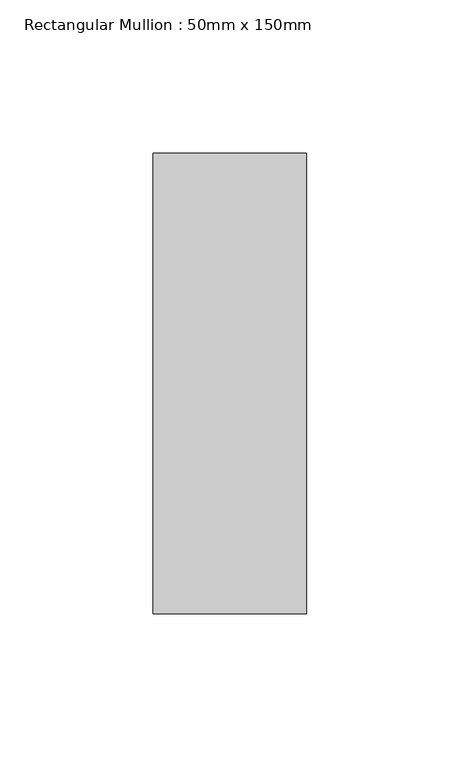
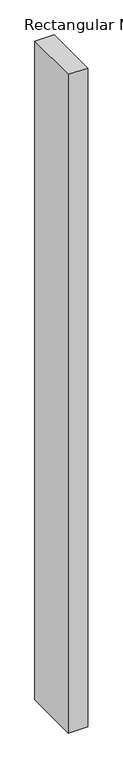
"""IFC4 building model written with IfcOpenShell, lengths in millimetres: member geometry, Rectangular Mullion : 50mm x 150mm."""

from ifc_helpers import new_model, si_unit, frame, origin, place, context, project, spatial, polyline, outline, extrude, source, transform, mapped, element, save


def rectangular_mullion_50mm_x_150mm_16fd62e7(model_context):
    return source(origin(), model_context, "Body", "SweptSolid", [
        extrude(outline(polyline([(25.0, 75.0), (25.0, -75.0), (-25.0, -75.0), (-25.0, 75.0), (25.0, 75.0)])), frame((0.0, 0.0, -1805.0000003), z_axis=(0.0, 0.0, 1.0), x_axis=(1.0, 0.0, 0.0)), (0.0, 0.0, 1.0), 1805.0000003),
    ])


if __name__ == "__main__":
    model = new_model("IFC4")
    model_context = context("Model", 3, world=origin())
    ifc_project = project(units=[si_unit("LENGTHUNIT", "METRE", prefix="MILLI")], contexts=[model_context])
    site = spatial("IfcSite", under=ifc_project)
    building = spatial("IfcBuilding", under=site)
    placement = place(None, origin())
    rectangular_mullion_50mm_x_150mm_shape = rectangular_mullion_50mm_x_150mm_16fd62e7(model_context)
    element("IfcMember", 1, ObjectType="Rectangular Mullion : 50mm x 150mm", at=placement, inside=building, context=model_context, shape_type="MappedRepresentation", body=[
        mapped(rectangular_mullion_50mm_x_150mm_shape, transform((0.0, 0.0, 0.0), x_axis=(1.0, 0.0, 0.0), y_axis=(0.0, 1.0, 0.0), z_axis=(0.0, 0.0, 1.0))),
    ])
    save(model, "model.ifc")

# Revit data of these elements
# Type "Rectangular Mullion : 50mm x 150mm"
#   built-in parameter 1007304 = 0.492126 (stored number, unit not read)
#   built-in parameter 1007301 = 0.082021 (stored number, unit not read)
#   built-in parameter 1007300 = 0.082021 (stored number, unit not read)
# Element 1 (IfcMember, "Rectangular Mullion : 50mm x 150mm")
#   Materials on its faces: "Aluminum"
# Materials
#   "Aluminum": class "Metal", colour RGB 244 244 244, transparency 0, Description = "Aluminum 6061", Cost = 0
